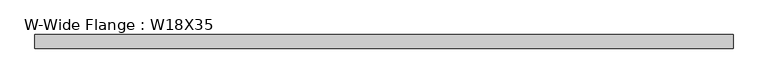
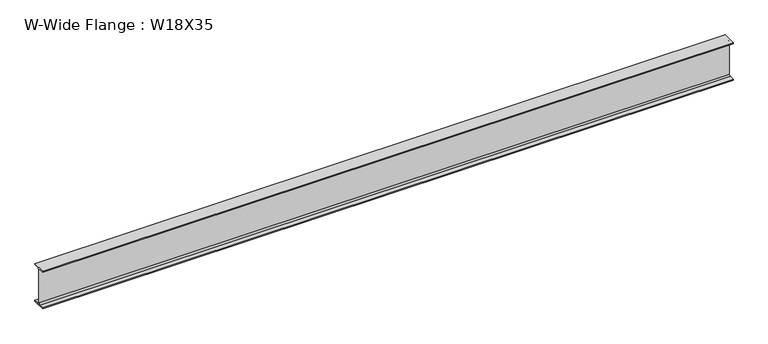
"""IFC4 building model written with IfcOpenShell, lengths in millimetres: beam geometry, W-Wide Flange : W18X35."""

from ifc_helpers import new_model, si_unit, point, frame, frame_2d, origin, place, context, project, spatial, polyline, circle_curve, trimmed, segment, composite_curve, outline, extrude, source, transform, mapped, element, save


def w_wide_flange_w18x35_45faa4ab(model_context):
    return source(origin(), model_context, "Body", "SweptSolid", [
        extrude(outline(composite_curve([segment(polyline([(76.2, -213.995), (76.2, -224.79), (-76.2, -224.79), (-76.2, -213.995), (-21.59, -213.995)]), True, "CONTINUOUS"), segment(trimmed(circle_curve(frame_2d((-21.59, -196.215)), 17.78), [point((-21.59, -213.995))], [point((-3.81, -196.215))], True, "CARTESIAN"), True, "CONTINUOUS"), segment(polyline([(-3.81, -196.215), (-3.81, 196.215)]), True, "CONTINUOUS"), segment(trimmed(circle_curve(frame_2d((-21.59, 196.215)), 17.78), [point((-3.81, 196.215))], [point((-21.59, 213.995))], True, "CARTESIAN"), True, "CONTINUOUS"), segment(polyline([(-21.59, 213.995), (-76.2, 213.995), (-76.2, 224.79), (76.2, 224.79), (76.2, 213.995), (21.59, 213.995)]), True, "CONTINUOUS"), segment(trimmed(circle_curve(frame_2d((21.59, 196.215)), 17.78), [point((21.59, 213.995))], [point((3.81, 196.215))], True, "CARTESIAN"), True, "CONTINUOUS"), segment(polyline([(3.81, 196.215), (3.81, -196.215)]), True, "CONTINUOUS"), segment(trimmed(circle_curve(frame_2d((21.59, -196.215)), 17.78), [point((3.81, -196.215))], [point((21.59, -213.995))], True, "CARTESIAN"), True, "CONTINUOUS"), segment(polyline([(21.59, -213.995), (76.2, -213.995)]), True, "CONTINUOUS")], self_intersect=False)), frame((-3911.6, 0.0, 0.0), z_axis=(1.0, 0.0, 0.0), x_axis=(0.0, 1.0, 0.0)), (0.0, 0.0, 1.0), 7823.2),
    ])


if __name__ == "__main__":
    model = new_model("IFC4")
    model_context = context("Model", 3, world=origin())
    ifc_project = project(units=[si_unit("LENGTHUNIT", "METRE", prefix="MILLI")], contexts=[model_context])
    site = spatial("IfcSite", under=ifc_project)
    building = spatial("IfcBuilding", under=site)
    placement = place(None, origin())
    w_wide_flange_w18x35_shape = w_wide_flange_w18x35_45faa4ab(model_context)
    element("IfcBeam", 1, ObjectType="W-Wide Flange : W18X35", at=placement, inside=building, context=model_context, shape_type="MappedRepresentation", body=[
        mapped(w_wide_flange_w18x35_shape, transform((0.0, 0.0, 0.0), x_axis=(1.0, 0.0, 0.0), y_axis=(0.0, 1.0, 0.0), z_axis=(0.0, 0.0, 1.0))),
    ])
    save(model, "model.ifc")

# Revit data of these elements
# Type "W-Wide Flange : W18X35"
#   Assembly Code = "B10"
#   W = 35
#   Length [instance default] = 5' - 0"
#   bf = 0' - 6"
#   d = 1' - 5.7"
#   k = 0' - 1 1/8"
#   k2 = 0' - 0.7"
#   tf = 0' - 0.425"
#   tw = 0' - 0.3"
#   A = 0.0715278 SF
#   Structural Material [instance default] = Steel ASTM A992
# Element 1 (IfcBeam, "W-Wide Flange : W18X35")
#   Materials on its faces: "Steel ASTM A992"
# Materials
#   "Steel ASTM A992": class "Metal", colour RGB 199 199 199, transparency 0, Description = "Structural steel 50ksi", Cost = 0
